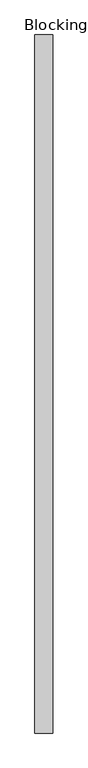
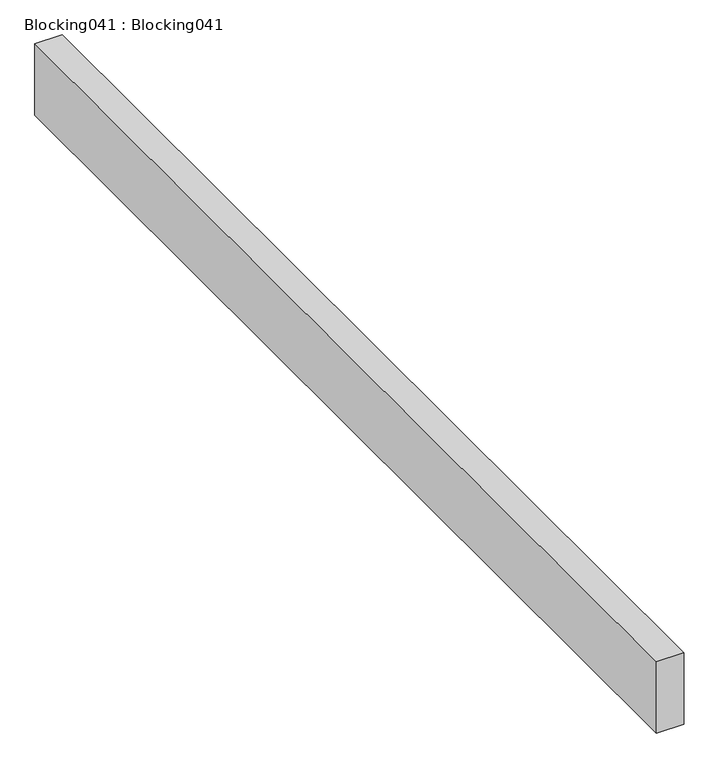
"""IFC4 building model written with IfcOpenShell, lengths in millimetres: proxy geometry, Blocking041 : Blocking041."""

from ifc_helpers import new_model, si_unit, frame, origin, place, context, project, spatial, polyline, outline, extrude, source, transform, mapped, element, save


def blocking041_blocking041_7534bca0(model_context):
    return source(origin(), model_context, "Body", "SweptSolid", [
        extrude(outline(polyline([(-4924.9038825, -1052.8908936), (-4975.7038825, -1052.8908936), (-4975.7038825, 947.1091064), (-4924.9038825, 947.1091064), (-4924.9038825, -1052.8908936)])), frame((0.0, 0.0, 39579.2960083), z_axis=(0.0, 0.0, 1.0), x_axis=(1.0, 0.0, 0.0)), (0.0, 0.0, 1.0), 139.7),
    ])


if __name__ == "__main__":
    model = new_model("IFC4")
    model_context = context("Model", 3, world=origin())
    ifc_project = project(units=[si_unit("LENGTHUNIT", "METRE", prefix="MILLI")], contexts=[model_context])
    site = spatial("IfcSite", under=ifc_project)
    building = spatial("IfcBuilding", under=site)
    placement = place(None, origin())
    blocking041_blocking041_shape = blocking041_blocking041_7534bca0(model_context)
    element("IfcBuildingElementProxy", 1, Name="Blocking041 : Blocking041", ObjectType="Blocking041 : Blocking041", at=placement, inside=building, context=model_context, shape_type="MappedRepresentation", body=[
        mapped(blocking041_blocking041_shape, transform((0.0, 0.0, 0.0), x_axis=(1.0, 0.0, 0.0), y_axis=(0.0, 1.0, 0.0), z_axis=(0.0, 0.0, 1.0))),
    ])
    save(model, "model.ifc")

# Revit data of these elements
# Type "Blocking041 : Blocking041"
#   NameOverride = "Blocking041"
# Element 1 (IfcBuildingElementProxy, "Blocking041 : Blocking041")
#   Materials on its faces: "WOOD BLOCKING AS REQUIRED"
# Materials
#   "WOOD BLOCKING AS REQUIRED": class "Unassigned", colour RGB 166 124 85, transparency 0, Cost = 0
